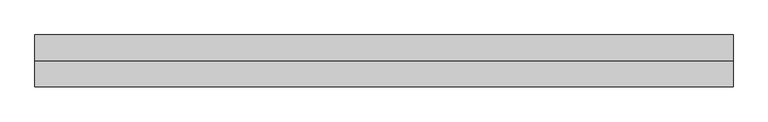
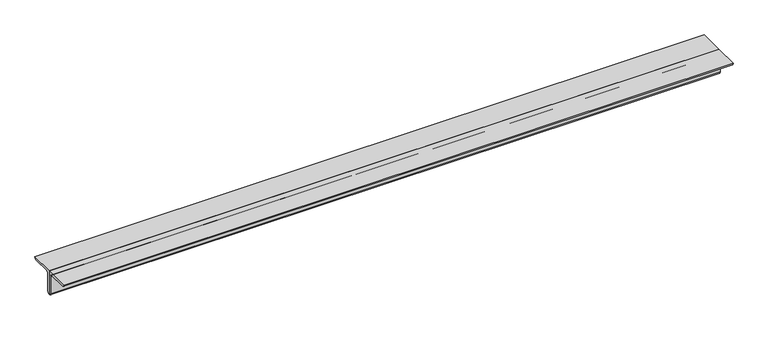
"""IFC4 building model written with IfcOpenShell, lengths in millimetres: member geometry, 0123_Steel Framing_2Ls-KSD3502 : H_SB_AR_S04_2Ls-130x130x12_VBR1."""

from ifc_helpers import new_model, si_unit, point, frame, frame_2d, origin, place, context, project, spatial, polyline, circle_curve, trimmed, segment, composite_curve, outline, extrude, source, transform, mapped, element, save


def member_96e87236(model_context):
    return source(origin(), model_context, "Body", "SweptSolid", [
        extrude(outline(composite_curve([segment(polyline([(0.0, 36.4), (130.0, 36.4)]), True, "CONTINUOUS"), segment(trimmed(circle_curve(frame_2d((118.0, 36.4)), 12.0), [point((130.0, 36.4))], [point((118.0, 24.4))], False, "CARTESIAN"), True, "CONTINUOUS"), segment(polyline([(118.0, 24.4), (24.0, 24.4)]), True, "CONTINUOUS"), segment(trimmed(circle_curve(frame_2d((24.0, 12.4)), 12.0), [point((24.0, 24.4))], [point((12.0, 12.4))], True, "CARTESIAN"), True, "CONTINUOUS"), segment(polyline([(12.0, 12.4), (12.0, -81.6)]), True, "CONTINUOUS"), segment(trimmed(circle_curve(frame_2d((0.0, -81.6)), 12.0), [point((12.0, -81.6))], [point((0.0, -93.6))], False, "CARTESIAN"), True, "CONTINUOUS"), segment(polyline([(0.0, -93.6), (0.0, 36.4)]), True, "CONTINUOUS")], self_intersect=False)), frame((-1749.149537, 0.0, 0.0), z_axis=(1.0, 0.0, 0.0), x_axis=(0.0, 1.0, 0.0)), (0.0, 0.0, 1.0), 3498.299074),
        extrude(outline(composite_curve([segment(polyline([(0.0, 36.4), (0.0, -93.6)]), True, "CONTINUOUS"), segment(trimmed(circle_curve(frame_2d((0.0, -81.6)), 12.0), [point((0.0, -93.6))], [point((-12.0, -81.6))], False, "CARTESIAN"), True, "CONTINUOUS"), segment(polyline([(-12.0, -81.6), (-12.0, 12.4)]), True, "CONTINUOUS"), segment(trimmed(circle_curve(frame_2d((-24.0, 12.4)), 12.0), [point((-12.0, 12.4))], [point((-24.0, 24.4))], True, "CARTESIAN"), True, "CONTINUOUS"), segment(polyline([(-24.0, 24.4), (-118.0, 24.4)]), True, "CONTINUOUS"), segment(trimmed(circle_curve(frame_2d((-118.0, 36.4)), 12.0), [point((-118.0, 24.4))], [point((-130.0, 36.4))], False, "CARTESIAN"), True, "CONTINUOUS"), segment(polyline([(-130.0, 36.4), (0.0, 36.4)]), True, "CONTINUOUS")], self_intersect=False)), frame((-1749.149537, 0.0, 0.0), z_axis=(1.0, 0.0, 0.0), x_axis=(0.0, 1.0, 0.0)), (0.0, 0.0, 1.0), 3498.299074),
    ])


if __name__ == "__main__":
    model = new_model("IFC4")
    model_context = context("Model", 3, world=origin())
    ifc_project = project(units=[si_unit("LENGTHUNIT", "METRE", prefix="MILLI")], contexts=[model_context])
    site = spatial("IfcSite", under=ifc_project)
    building = spatial("IfcBuilding", under=site)
    placement = place(None, origin())
    member_shape = member_96e87236(model_context)
    element("IfcMember", 1, ObjectType="0123_Steel Framing_2Ls-KSD3502 : H_SB_AR_S04_2Ls-130x130x12_VBR1", at=placement, inside=building, context=model_context, shape_type="MappedRepresentation", body=[
        mapped(member_shape, transform((0.0, 0.0, 0.0), x_axis=(1.0, 0.0, 0.0), y_axis=(0.0, 1.0, 0.0), z_axis=(0.0, 0.0, 1.0))),
    ])
    save(model, "model.ifc")

# Revit data of these elements
# Type "0123_Steel Framing_2Ls-KSD3502 : H_SB_AR_S04_2Ls-130x130x12_VBR1"
#   Assembly Code = "B10"
#   Legs = "SLBB"
#   W = 8.97
#   Perimeter = 1.04 m²/m
#   Nominal Weight = 46.80 kgf/m
#   Length [instance default] = 1000 mm
#   Space = 0 mm
#   b = 130 mm
#   d = 130 mm
#   t = 12 mm
#   y = 36.4 mm
#   A = 0.005952 m²
#   Structural Material [instance default] = Steel ASTM A36
# Element 1 (IfcMember, "0123_Steel Framing_2Ls-KSD3502 : H_SB_AR_S04_2Ls-130x130x12_VBR1")
#   Structural Material = Steel, 45-345
#   Materials on its faces: "Steel, 45-345"
# Materials
#   "Steel ASTM A36": class "Metal", colour RGB 199 199 199, transparency 0, Description = "Structural steel, ASTM A36 Grade B, mill finish", Cost = 0
#   "Steel, 45-345": class "Metal", colour RGB 189 187 185, transparency 0, Description = "Steel 345 MPa", Cost = 0
